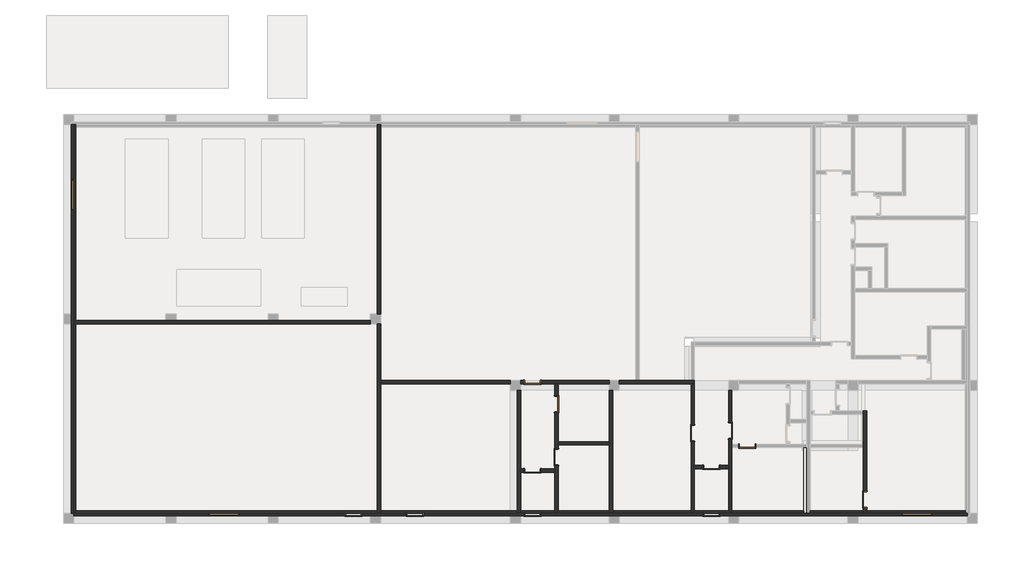
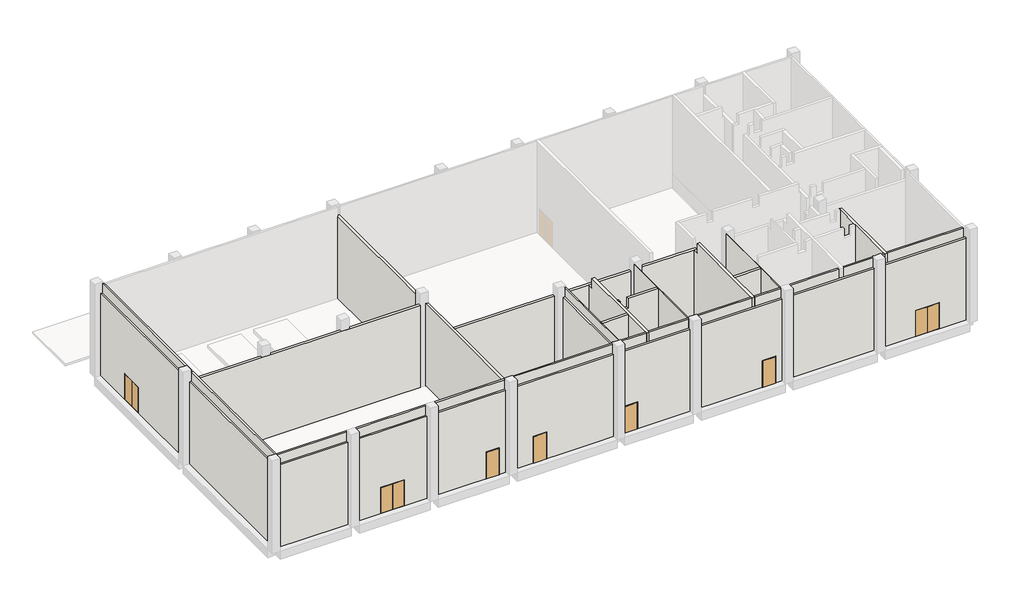
# One storey, part 1 of 4: 31 walls, 16 doors.
# Revit data of these elements (continued)
# Type "Double Door_Steel : H_DR_AR B12_Door_Double SD 02"
#   Type Mark = "FSD"
#   프레임 = ""
#   철물 = ""
#   유리/마감 = ""
#   위치/개소 = ""
#   부호 = "1/SD"
#   문번호 = ""
#   문기호 = "SD"
#   Analytic Construction = "<None>"
#   Height = 2100 mm
#   Width = 1800 mm
#   Define Thermal Properties by = 1
#   문 틀 = none
#   문 = none
#   Function = (empty or 0)
#   Assembly Code = ""
#   Wall Closure = (empty or 0)
# Type "Double Door_Steel : H_DR_AR B12_Door_Double FSD 02"
#   Type Mark = "FRD"
#   프레임 = ""
#   철물 = ""
#   유리/마감 = ""
#   위치/개소 = ""
#   부호 = "1/SD"
#   문번호 = ""
#   문기호 = "SD"
#   Analytic Construction = "<None>"
#   Height = 2100 mm
#   Width = 1800 mm
#   Define Thermal Properties by = 1
#   문 틀 = none
#   문 = none
#   Function = (empty or 0)
#   Assembly Code = ""
#   Wall Closure = (empty or 0)
# Type "Single Door_Steel : H_DR_AR B12_Door_Single FSD 01"
#   Type Mark = "FRD"
#   Analytic Construction = "<None>"
#   프레임 투영 외부. = 25 mm
#   프레임 투영 내부. = 25 mm
#   프레임 폭 = 75 mm
#   Height = 2160 mm
#   Width = 1020 mm
#   Define Thermal Properties by = 1
#   문 패널 = none
#   문 프레임 = none
#   Function = (empty or 0)
#   Wall Closure = (empty or 0)
# Type "H_WA_AR B02_Ext Wall RC-AG_EW5"
#   Type Comments = "AG"
#   Type Mark = "W1"
#   H_Rebar Ratio = 0.12
#   Layers, outside or top first: 0 mm no material (function 100); 0 mm no material (function 100); 150 mm no material (function 1); 0 mm no material (function 100); 0 mm no material (function 100); 0 mm no material (function 100)
# Type "H_WA_AR_B02_Ext Wall_RC_T200_W2"
#   Type Comments = "AG"
#   Type Mark = "W2"
#   H_Rebar Ratio = 0.12
#   Layers, outside or top first: 200 mm no material (function 1)
# Type "H_WA_AR B02_Int Wall MA_IW1 T200"
#   Type Comments = ""
#   Layers, outside or top first: 200 mm "00_Masonry_Conc. Block" (function 1)
# Type "H_WA_AR B02_Ext Wall DY-IN_EW1_VB"
#   Type Comments = "구조_콘크리트"
#   Layers, outside or top first: 126 mm "Rock Wool" (function 1)
# Element 1 (IfcDoor, "Double Door_Steel : H_DR_AR B12_Door_Double SD 02")
#   Frame Material = "ST"
#   H_Door Style Name = "Steel Door_Double_Normal_Fire Rating"
#   H_Door_Leaf = "ST"
#   H_Door_Vision = "-"
#   H_Door_Panic = "-"
#   H_Door_Style Remark = ""
#   H_Door_Type = "B1"
#   H_Door_Louver = "-"
#   H_Door Style No = 212_FSD_DD_N_F
#   Phase Created = New Construction
# Elements 2, 3 (IfcDoor, "Double Door_Steel : H_DR_AR B12_Door_Double FSD 02")
#   Frame Material = "ST"
#   H_Door Style Name = "Steel Door_Double_Normal_Fire Rating"
#   H_Door_Leaf = "ST"
#   H_Door_Vision = "-"
#   H_Door_Panic = "-"
#   H_Door_Style Remark = ""
#   H_Door_Type = "B1"
#   H_Door_Louver = "-"
#   H_Door Style No = 212_FSD_DD_N_F
#   Phase Created = New Construction
# Elements 4, 5, 6, 7, 8, 10, 11, 12, 13, 14, 15, 16 (IfcDoor, "Single Door_Steel : H_DR_AR B12_Door_Single FSD 01")
#   Frame Material = "ST"
#   H_Door Style Name = "Steel Door_Single_Normal_Fire Rating"
#   H_Door_Leaf = "ST"
#   H_Door_Vision = "-"
#   H_Door_Panic = "-"
#   H_Door_Style Remark = ""
#   H_Door_Type = "A1"
#   H_Door_Louver = "-"
#   H_Door Style No = 112_FSD_SD_N_F
#   Phase Created = New Construction
# Element 9 (IfcDoor, "Single Door_Steel : H_DR_AR B12_Door_Single FSD 01")
#   Frame Material = "WD"
#   H_Door Style Name = "Wood Door_Single_Normal"
#   H_Door_Leaf = "WD"
#   H_Door_Vision = "-"
#   H_Door_Panic = "-"
#   H_Door_Style Remark = ""
#   H_Door_Type = "A1"
#   H_Door_Louver = "-"
#   H_Door Style No = 181_WD_SD_N
#   Phase Created = New Construction
# Elements 17, 18 (IfcWall, "H_WA_AR B02_Ext Wall RC-AG_EW5")
#   H_Wall Style Name = "Concrete Wall+Acrylic Emulsion Paint on Fair Faced Concrete+Insulation"
#   H_Wall_Style Remark = ""
#   Top Offset = 0 mm
#   Base Offset = 0 mm
#   wall height = 7500.038 mm
#   H_Wall Style No = EW512A_CO
#   Phase Created = New Construction
#   Base Constraint = TOC(GF)
#   Top Constraint = TOC
#   Materials on its faces: "00_Concrete_Reinf. Conc."
# Elements 19, 20, 21 (IfcWall, "H_WA_AR_B02_Ext Wall_RC_T200_W2")
#   H_Wall Style Name = "Concrete Wall"
#   H_Wall_Style Remark = ""
#   Top Offset = 0 mm
#   Base Offset = 0 mm
#   wall height = 1000 mm
#   H_Wall Style No = IW311_CO
#   Phase Created = New Construction
#   Base Constraint = TOC(GF)
#   Top Constraint = TOC(GF-1)
#   Materials on its faces: "00_Concrete_Reinf. Conc."
# Elements 22, 23, 24, 25, 26, 27, 28, 29, 30, 31, 32, 33, 34, 35, 36 (IfcWall, "H_WA_AR B02_Int Wall MA_IW1 T200")
#   H_Wall Style Name = "Block Wall"
#   H_Wall_Style Remark = ""
#   Top Offset = 0 mm
#   Base Offset = 0 mm
#   wall height = 7500.038 mm
#   H_Wall Style No = IW211_BL
#   Phase Created = New Construction
#   Base Constraint = TOC(GF)
#   Top Constraint = TOC
#   Materials on its faces: "00_Masonry_Conc. Block"
# Elements 37, 38, 39, 40, 41, 42, 43, 44, 45, 46, 47 (IfcWall, "H_WA_AR B02_Ext Wall DY-IN_EW1_VB")
#   Top Offset = 0 mm
#   Base Offset = 0 mm
#   wall height = 7500.038 mm
#   Phase Created = New Construction
#   Base Constraint = TOC(GF)
#   Top Constraint = TOC
#   Materials on its faces: "Rock Wool"
# Materials
#   "00_Masonry_Conc. Block": class "Concrete", colour RGB 180 180 180, transparency 0, Description = "Conc. Block", Cost = 0, Image = Brick_Uniform_12inch_Running_Gray.png
#   "Rock Wool": class "Generic", colour RGB 120 120 120, transparency 0, Description = "Rock Wool", Cost = 0
#   "00_Concrete_Reinf. Conc.": class "Concrete", colour RGB 176 176 176, transparency 0, Description = "Reinf. Conc.", Cost = 0, Image = Concrete.Cast-In-Place.Flat.Polished.Grey.jpg
# Room at (9212.5, -2162.5) mm, phase "New Construction", upper level "TOC(GF)", upper offset 10500 mm, lower offset 0 mm
#   Comments = ""
#   Base Finish = "Epoxy Paint"
#   Ceiling Finish = "Acrylic Emulsion Paint"
#   Wall Finish = "Acrylic Emulsion Paint"
#   Floor Finish = "Epoxy Paint on Hardener Finish(Powder Type)"
#   Number = "101"
#   Name = "MECHANICAL ROOM"
#   H_Floor Base Material = "Concrete Slab"
#   H_Floor Finish Remark = "-"
#   H_Skirt Base Material = "Same as Wall"
#   H_Skirt Finish Remark = "-"
#   H_Wall Base Material = "Masonry Wall / Cement Plaster"
#   H_Wall Finish Remark = "-"
#   H_Ceiling Base Material = "Concrete Slab / Fair Faced Concrete"
#   H_Ceiling Finish Remark = "-"
#   Floor Finish Style No = FF331_HD_EP
#   Skirt Finish Style No = FB121_PA_EP
#   Wall Finish Style No = FW102_PA_AE
#   Ceiling Finish Style No = FC101_PA_AE
# Room at (9212.5, -13637.5) mm, phase "New Construction", upper level "TOC(GF)", upper offset 10500 mm, lower offset 0 mm
#   Comments = ""
#   Base Finish = "Epoxy Paint"
#   Ceiling Finish = "Acrylic Emulsion Paint"
#   Wall Finish = "Acrylic Emulsion Paint"
#   Floor Finish = "Non-Slip Epoxy Paint"
#   Number = "112"
#   Name = "ELECTRICAL ROOM(SS08)"
#   H_Floor Base Material = "Concrete Slab / Screed"
#   H_Floor Finish Remark = "-"
#   H_Skirt Base Material = "Same as Wall"
#   H_Skirt Finish Remark = "-"
#   H_Wall Base Material = "Masonry Wall / Cement Plaster"
#   H_Wall Finish Remark = "-"
#   H_Ceiling Base Material = "Concrete Slab / Fair Faced Concrete"
#   H_Ceiling Finish Remark = "-"
#   Floor Finish Style No = FF162_PA_EP
#   Skirt Finish Style No = FB121_PA_EP
#   Wall Finish Style No = FW102_PA_AE
#   Ceiling Finish Style No = FC101_PA_AE
# Room at (22300, -15387.5) mm, phase "New Construction", upper level "TOC(GF)", upper offset 10500 mm, lower offset 0 mm
#   Comments = ""
#   Base Finish = "Acid Resistant Ceramic Tile"
#   Ceiling Finish = "Acrylic Emulsion Paint"
#   Wall Finish = "Acid Resistant Paint"
#   Floor Finish = "Acid Resistant Ceramic Tile"
#   Number = "114"
#   Name = "BATTERY ROOM"
#   H_Floor Base Material = "Concrete Slab / Screed / Liquid Waterproofing"
#   H_Floor Finish Remark = "-"
#   H_Skirt Base Material = "Same as Wall"
#   H_Skirt Finish Remark = "-"
#   H_Wall Base Material = "Masonry Wall / Cement Plaster"
#   H_Wall Finish Remark = "-"
#   H_Ceiling Base Material = "Concrete Slab / Fair Faced Concrete"
#   H_Ceiling Finish Remark = "-"
#   Floor Finish Style No = FF222_TL_AC
#   Skirt Finish Style No = FB221_TL_AC
#   Wall Finish Style No = FW122_PA_AR
#   Ceiling Finish Style No = FC101_PA_AE
# Room at (49387.5, -3982.5) mm, phase "New Construction", upper level "TOC(GF)", upper offset 10500 mm, lower offset 0 mm
#   Comments = ""
#   Base Finish = "Coved Vinyl Tile"
#   Ceiling Finish = "Suspended Moisture Resistant Tiled Ceiling (M-Bar)"
#   Wall Finish = "Acrylic Emulsion Paint"
#   Floor Finish = "Vinyl Tile"
#   Number = "108"
#   Name = "BREAK ROOM"
#   H_Floor Base Material = "Concrete Slab / Screed"
#   H_Floor Finish Remark = "-"
#   H_Skirt Base Material = "Same as Wall"
#   H_Skirt Finish Remark = "-"
#   H_Wall Base Material = "Masonry Wall / Cement Plaster"
#   H_Wall Finish Remark = "-"
#   H_Ceiling Base Material = "Concrete Slab / Fair Faced Concrete"
#   H_Ceiling Finish Remark = "-"
#   H_Room H or CH = 2700 mm
#   Floor Finish Style No = FF232_TL_VN
#   Skirt Finish Style No = FB231_TL_VL
#   Wall Finish Style No = FW102_PA_AE
#   Ceiling Finish Style No = FC541_SC_MT
# Room at (50137.5, 912.5) mm, phase "New Construction", upper level "TOC(GF)", upper offset 10500 mm, lower offset 0 mm
#   Comments = ""
#   Base Finish = "Coved Vinyl Tile"
#   Ceiling Finish = "Suspended Acoustic Tiled Ceiling (M-Bar)"
#   Wall Finish = "Acrylic Emulsion Paint"
#   Floor Finish = "Vinyl Tile"
#   Number = "106"
#   Name = "SHIFT SUPERVISOR/DAY SUPERVISOR"
#   H_Floor Base Material = "Concrete Slab / Screed"
#   H_Floor Finish Remark = "-"
#   H_Skirt Base Material = "Same as Wall"
#   H_Skirt Finish Remark = "-"
#   H_Wall Base Material = "Masonry Wall / Cement Plaster"
#   H_Wall Finish Remark = "-"
#   H_Ceiling Base Material = "Concrete Slab / Fair Faced Concrete"
#   H_Ceiling Finish Remark = "-"
#   H_Room H or CH = 2700 mm
#   Floor Finish Style No = FF232_TL_VN
#   Skirt Finish Style No = FB231_TL_VL
#   Wall Finish Style No = FW102_PA_AE
#   Ceiling Finish Style No = FC531_SC_AT
# Room at (41100, -17262.5) mm, phase "New Construction", upper level "TOC(GF)", upper offset 10500 mm, lower offset 0 mm
#   Comments = ""
#   Base Finish = "Coved Ceramic Tile"
#   Ceiling Finish = "Suspended Moisture Resistant Tiled Ceiling (M-Bar)"
#   Wall Finish = "Glazed Ceramic Tile (≤2100) / Acrylic Emulsion Paint (>2100)"
#   Floor Finish = "Non-Slip Unglazed Ceramic Tile"
#   Number = "122"
#   Name = "TOILETS"
#   H_Floor Base Material = "Concrete Slab / Screed / Liquid Waterproofing"
#   H_Floor Finish Remark = "ex) 150x150x6T"
#   H_Skirt Base Material = "Same as Wall"
#   H_Skirt Finish Remark = "-"
#   H_Wall Base Material = "Masonry Wall"
#   H_Wall Finish Remark = ""
#   H_Ceiling Base Material = "Concrete Slab / Fair Faced Concrete"
#   H_Ceiling Finish Remark = "-"
#   H_Room H or CH = 2700 mm
#   Floor Finish Style No = FF202_TL_UC
#   Skirt Finish Style No = FB211_TL_CC
#   Wall Finish Style No = FW212C_TL_GC
#   Ceiling Finish Style No = FC541_SC_MT
# Room at (45050, -17262.5) mm, phase "New Construction", upper level "TOC(GF)", upper offset 10500 mm, lower offset 0 mm
#   Comments = ""
#   Base Finish = "Coved Vinyl Tile"
#   Ceiling Finish = "Suspended Acoustic Tiled Ceiling (M-Bar)"
#   Wall Finish = "Acrylic Emulsion Paint"
#   Floor Finish = "Vinyl Tile"
#   Number = "124"
#   Name = "STORE"
#   H_Floor Base Material = "Concrete Slab / Screed"
#   H_Floor Finish Remark = "-"
#   H_Skirt Base Material = "Same as Wall"
#   H_Skirt Finish Remark = "-"
#   H_Wall Base Material = "Masonry Wall / Cement Plaster"
#   H_Wall Finish Remark = "-"
#   H_Ceiling Base Material = "Concrete Slab / Fair Faced Concrete"
#   H_Ceiling Finish Remark = "-"
#   H_Room H or CH = 2700 mm
#   Floor Finish Style No = FF232_TL_VN
#   Skirt Finish Style No = FB231_TL_VL
#   Wall Finish Style No = FW102_PA_AE
#   Ceiling Finish Style No = FC531_SC_AT
# Room at (37700, -17887.5) mm, phase "New Construction", upper level "TOC(GF)", upper offset 10500 mm, lower offset 0 mm
#   Comments = ""
#   Base Finish = "Coved Vinyl Tile"
#   Ceiling Finish = "Suspended Acoustic Tiled Ceiling (M-Bar)"
#   Wall Finish = "Acrylic Emulsion Paint"
#   Floor Finish = "Vinyl Tile"
#   Number = "119"
#   Name = "AIR LOCK"
#   H_Floor Base Material = "Concrete Slab / Screed"
#   H_Floor Finish Remark = "-"
#   H_Skirt Base Material = "Same as Wall"
#   H_Skirt Finish Remark = "-"
#   H_Wall Base Material = "Masonry Wall / Cement Plaster"
#   H_Wall Finish Remark = "-"
#   H_Ceiling Base Material = "Concrete Slab / Fair Faced Concrete"
#   H_Ceiling Finish Remark = "-"
#   H_Room H or CH = 2700 mm
#   Floor Finish Style No = FF232_TL_VN
#   Skirt Finish Style No = FB231_TL_VL
#   Wall Finish Style No = FW102_PA_AE
#   Ceiling Finish Style No = FC531_SC_AT
# Room at (27500, -17987.5) mm, phase "New Construction", upper level "TOC(GF)", upper offset 10500 mm, lower offset 0 mm
#   Comments = ""
#   Base Finish = "Coved Vinyl Tile"
#   Ceiling Finish = "Suspended Acoustic Tiled Ceiling (M-Bar)"
#   Wall Finish = "Acrylic Emulsion Paint"
#   Floor Finish = "Vinyl Tile"
#   Number = "117"
#   Name = "AIR LOCK"
#   H_Floor Base Material = "Concrete Slab / Screed"
#   H_Floor Finish Remark = "-"
#   H_Skirt Base Material = "Same as Wall"
#   H_Skirt Finish Remark = "-"
#   H_Wall Base Material = "Masonry Wall / Cement Plaster"
#   H_Wall Finish Remark = "-"
#   H_Ceiling Base Material = "Concrete Slab / Fair Faced Concrete"
#   H_Ceiling Finish Remark = "-"
#   H_Room H or CH = 2700 mm
#   Floor Finish Style No = FF232_TL_VN
#   Skirt Finish Style No = FB231_TL_VL
#   Wall Finish Style No = FW102_PA_AE
#   Ceiling Finish Style No = FC531_SC_AT
# Room at (27500, -14100) mm, phase "New Construction", upper level "TOC(GF)", upper offset 10500 mm, lower offset 0 mm
#   Comments = ""
#   Base Finish = "Coved Vinyl Tile"
#   Ceiling Finish = "Suspended Acoustic Tiled Ceiling (M-Bar)"
#   Wall Finish = "Acrylic Emulsion Paint"
#   Floor Finish = "Vinyl Tile"
#   Number = "116"
#   Name = "CORRIDOR"
#   H_Floor Base Material = "Concrete Slab / Screed"
#   H_Floor Finish Remark = "-"
#   H_Skirt Base Material = "Same as Wall"
#   H_Skirt Finish Remark = "-"
#   H_Wall Base Material = "Masonry Wall / Cement Plaster"
#   H_Wall Finish Remark = "-"
#   H_Ceiling Base Material = "Concrete Slab / Fair Faced Concrete"
#   H_Ceiling Finish Remark = "-"
#   H_Room H or CH = 2700 mm
#   Floor Finish Style No = FF232_TL_VN
#   Skirt Finish Style No = FB231_TL_VL
#   Wall Finish Style No = FW102_PA_AE
#   Ceiling Finish Style No = FC531_SC_AT
# Room at (30200, -17187.5) mm, phase "New Construction", upper level "TOC(GF)", upper offset 10500 mm, lower offset 0 mm
#   Comments = ""
#   Base Finish = "Coved Vinyl Tile"
#   Ceiling Finish = "Acrylic Emulsion Paint"
#   Wall Finish = "2-COATS OF NON-CONDUCTIVE & FIRE RETARTDANT WITH COLOR PAINT"
#   Floor Finish = "Vinyl Tile"
#   Number = "115"
#   Name = "TELECOMS ROOM"
#   H_Floor Base Material = "Concrete Slab / Screed"
#   H_Floor Finish Remark = "-"
#   H_Skirt Base Material = "Same as Wall"
#   H_Skirt Finish Remark = "-"
#   H_Wall Base Material = "Masonry Wall / Cement Plaster"
#   H_Wall Finish Remark = ""
#   H_Ceiling Base Material = "Concrete Slab / Fair Faced Concrete"
#   H_Ceiling Finish Remark = "-"
#   Floor Finish Style No = FF232_TL_VN
#   Skirt Finish Style No = FB231_TL_VL
#   Wall Finish Style No = FW182_PA_CF
#   Ceiling Finish Style No = FC101_PA_AE
# Room at (49387.5, -8082.5) mm, phase "New Construction", upper level "TOC(GF)", upper offset 10500 mm, lower offset 0 mm
#   Comments = ""
#   Base Finish = "Coved Vinyl Tile"
#   Ceiling Finish = "Suspended Acoustic Tiled Ceiling (M-Bar)"
#   Wall Finish = "Acrylic Emulsion Paint"
#   Floor Finish = "Carpet Tile"
#   Number = "111"
#   Name = "PRAYER ROOM"
#   H_Floor Base Material = "Concrete Slab / Steel Trowel Finish"
#   H_Floor Finish Remark = "-"
#   H_Skirt Base Material = "Same as Wall"
#   H_Skirt Finish Remark = "-"
#   H_Wall Base Material = "Masonry Wall / Cement Plaster"
#   H_Wall Finish Remark = "-"
#   H_Ceiling Base Material = "Concrete Slab / Fair Faced Concrete"
#   H_Ceiling Finish Remark = "-"
#   H_Room H or CH = 2700 mm
#   Floor Finish Style No = FF275_TL_CA
#   Skirt Finish Style No = FB231_TL_VL
#   Wall Finish Style No = FW102_PA_AE
#   Ceiling Finish Style No = FC531_SC_AT
# Room at (30200, -13300) mm, phase "New Construction", upper level "TOC(GF)", upper offset 10500 mm, lower offset 0 mm
#   Comments = ""
#   Base Finish = "Coved Vinyl Tile"
#   Ceiling Finish = "Suspended Acoustic Tiled Ceiling (M-Bar)"
#   Wall Finish = "Acrylic Emulsion Paint"
#   Floor Finish = "Vinyl Tile"
#   Number = "113"
#   Name = "STORE"
#   H_Floor Base Material = "Concrete Slab / Screed"
#   H_Floor Finish Remark = "-"
#   H_Skirt Base Material = "Same as Wall"
#   H_Skirt Finish Remark = "-"
#   H_Wall Base Material = "Masonry Wall / Cement Plaster"
#   H_Wall Finish Remark = "-"
#   H_Ceiling Base Material = "Concrete Slab / Fair Faced Concrete"
#   H_Ceiling Finish Remark = "-"
#   H_Room H or CH = 2700 mm
#   Floor Finish Style No = FF232_TL_VN
#   Skirt Finish Style No = FB231_TL_VL
#   Wall Finish Style No = FW102_PA_AE
#   Ceiling Finish Style No = FC531_SC_AT
# Room at (34200, -15387.5) mm, phase "New Construction", upper level "TOC(GF)", upper offset 10500 mm, lower offset 0 mm
#   Comments = ""
#   Base Finish = "Coved Vinyl Tile"
#   Ceiling Finish = "Suspended Acoustic Tiled Ceiling (M-Bar)"
#   Wall Finish = "Acrylic Emulsion Paint"
#   Floor Finish = "Vinyl Tile"
#   Number = "118"
#   Name = "DRIVERS LOUNGE"
#   H_Floor Base Material = "Concrete Slab / Screed"
#   H_Floor Finish Remark = "-"
#   H_Skirt Base Material = "Same as Wall"
#   H_Skirt Finish Remark = "-"
#   H_Wall Base Material = "Masonry Wall / Cement Plaster"
#   H_Wall Finish Remark = "-"
#   H_Ceiling Base Material = "Concrete Slab / Fair Faced Concrete"
#   H_Ceiling Finish Remark = "-"
#   H_Room H or CH = 2700 mm
#   Floor Finish Style No = FF232_TL_VN
#   Skirt Finish Style No = FB231_TL_VL
#   Wall Finish Style No = FW102_PA_AE
#   Ceiling Finish Style No = FC531_SC_AT
# Room at (48937.5, -15387.5) mm, phase "New Construction", upper level "TOC(GF)", upper offset 10500 mm, lower offset 0 mm
#   Comments = ""
#   Base Finish = "Epoxy Paint"
#   Ceiling Finish = "Acrylic Emulsion Paint"
#   Wall Finish = "Acrylic Emulsion Paint"
#   Floor Finish = "Non-Slip Epoxy Paint with Epoxy Hardener"
#   Number = "125"
#   Name = "MAINTENANCE WORKSHOP"
#   H_Floor Base Material = "Concrete Slab / Steel Trowel Finish"
#   H_Floor Finish Remark = "-"
#   H_Skirt Base Material = "Same as Wall"
#   H_Skirt Finish Remark = "-"
#   H_Wall Base Material = "Masonry Wall / Cement Plaster"
#   H_Wall Finish Remark = "-"
#   H_Ceiling Base Material = "Concrete Slab / Fair Faced Concrete"
#   H_Ceiling Finish Remark = "-"
#   Floor Finish Style No = FF351_HD_EP
#   Skirt Finish Style No = FB121_PA_EP
#   Wall Finish Style No = FW102_PA_AE
#   Ceiling Finish Style No = FC101_PA_AE
# Room at (51435, -9900) mm, phase "New Construction", upper level "TOC(GF)", upper offset 10500 mm, lower offset 0 mm
#   Comments = ""
#   Base Finish = "Coved Ceramic Tile"
#   Ceiling Finish = "Suspended Moisture Resistant Tiled Ceiling (M-Bar)"
#   Wall Finish = "Glazed Ceramic Tile (≤2100) / Acrylic Emulsion Paint (>2100)"
#   Floor Finish = "Non-Slip Unglazed Ceramic Tile"
#   Number = "110"
#   Name = "ABLUTIONS"
#   H_Floor Base Material = "Concrete Slab / Screed / Liquid Waterproofing"
#   H_Floor Finish Remark = "ex) 150x150x6T"
#   H_Skirt Base Material = "Same as Wall"
#   H_Skirt Finish Remark = "-"
#   H_Wall Base Material = "Masonry Wall"
#   H_Wall Finish Remark = ""
#   H_Ceiling Base Material = "Concrete Slab / Fair Faced Concrete"
#   H_Ceiling Finish Remark = "-"
#   H_Room H or CH = 2700 mm
#   Floor Finish Style No = FF202_TL_UC
#   Skirt Finish Style No = FB211_TL_CC
#   Wall Finish Style No = FW212C_TL_GC
#   Ceiling Finish Style No = FC541_SC_MT
# Room at (43535, -10780.912) mm, phase "New Construction", upper level "TOC(GF)", upper offset 10500 mm, lower offset 0 mm
#   Comments = ""
#   Base Finish = "Coved Vinyl Tile"
#   Ceiling Finish = "Suspended Acoustic Tiled Ceiling (M-Bar)"
#   Wall Finish = "Acrylic Emulsion Paint"
#   Floor Finish = "Vinyl Tile"
#   Number = "120"
#   Name = "CORRIDOR"
#   H_Floor Base Material = "Concrete Slab / Screed"
#   H_Floor Finish Remark = "-"
#   H_Skirt Base Material = "Same as Wall"
#   H_Skirt Finish Remark = "-"
#   H_Wall Base Material = "Masonry Wall / Cement Plaster"
#   H_Wall Finish Remark = "-"
#   H_Ceiling Base Material = "Concrete Slab / Fair Faced Concrete"
#   H_Ceiling Finish Remark = "-"
#   H_Room H or CH = 2700 mm
#   Floor Finish Style No = FF232_TL_VN
#   Skirt Finish Style No = FB231_TL_VL
#   Wall Finish Style No = FW102_PA_AE
#   Ceiling Finish Style No = FC531_SC_AT
# Room at (44850, 2237.5) mm, phase "New Construction", upper level "TOC(GF)", upper offset 10500 mm, lower offset 0 mm
#   Comments = ""
#   Base Finish = "Coved Vinyl Tile"
#   Ceiling Finish = "Suspended Acoustic Tiled Ceiling (M-Bar)"
#   Wall Finish = "Acrylic Emulsion Paint"
#   Floor Finish = "Vinyl Tile"
#   Number = "104"
#   Name = "AIR LOCK"
#   H_Floor Base Material = "Concrete Slab / Screed"
#   H_Floor Finish Remark = "-"
#   H_Skirt Base Material = "Same as Wall"
#   H_Skirt Finish Remark = "-"
#   H_Wall Base Material = "Masonry Wall / Cement Plaster"
#   H_Wall Finish Remark = "-"
#   H_Ceiling Base Material = "Concrete Slab / Fair Faced Concrete"
#   H_Ceiling Finish Remark = "-"
#   H_Room H or CH = 2700 mm
#   Floor Finish Style No = FF232_TL_VN
#   Skirt Finish Style No = FB231_TL_VL
#   Wall Finish Style No = FW102_PA_AE
#   Ceiling Finish Style No = FC531_SC_AT
# Room at (47500, 1612.5) mm, phase "New Construction", upper level "TOC(GF)", upper offset 10500 mm, lower offset 0 mm
#   Comments = ""
#   Base Finish = "Coved Vinyl Tile"
#   Ceiling Finish = "Suspended Acoustic Tiled Ceiling (M-Bar)"
#   Wall Finish = "Acrylic Emulsion Paint"
#   Floor Finish = "Vinyl Tile"
#   Number = "105"
#   Name = "LIBRARY"
#   H_Floor Base Material = "Concrete Slab / Screed"
#   H_Floor Finish Remark = "-"
#   H_Skirt Base Material = "Same as Wall"
#   H_Skirt Finish Remark = "-"
#   H_Wall Base Material = "Masonry Wall / Cement Plaster"
#   H_Wall Finish Remark = "-"
#   H_Ceiling Base Material = "Concrete Slab / Fair Faced Concrete"
#   H_Ceiling Finish Remark = "-"
#   H_Room H or CH = 2700 mm
#   Floor Finish Style No = FF232_TL_VN
#   Skirt Finish Style No = FB231_TL_VL
#   Wall Finish Style No = FW102_PA_AE
#   Ceiling Finish Style No = FC531_SC_AT
# Room at (45600, -4225) mm, phase "New Construction", upper level "TOC(GF)", upper offset 10500 mm, lower offset 0 mm
#   Comments = ""
#   Base Finish = "Coved Vinyl Tile"
#   Ceiling Finish = "Suspended Acoustic Tiled Ceiling (M-Bar)"
#   Wall Finish = "Acrylic Emulsion Paint"
#   Floor Finish = "Vinyl Tile"
#   Number = "107"
#   Name = "CORRIDOR"
#   H_Floor Base Material = "Concrete Slab / Screed"
#   H_Floor Finish Remark = "-"
#   H_Skirt Base Material = "Same as Wall"
#   H_Skirt Finish Remark = "-"
#   H_Wall Base Material = "Masonry Wall / Cement Plaster"
#   H_Wall Finish Remark = "-"
#   H_Ceiling Base Material = "Concrete Slab / Fair Faced Concrete"
#   H_Ceiling Finish Remark = "-"
#   H_Room H or CH = 2700 mm
#   Floor Finish Style No = FF232_TL_VN
#   Skirt Finish Style No = FB231_TL_VL
#   Wall Finish Style No = FW102_PA_AE
#   Ceiling Finish Style No = FC531_SC_AT
# Room at (38525, -3912.5) mm, phase "New Construction", upper level "TOC(GF)", upper offset 10500 mm, lower offset 0 mm
#   Comments = ""
#   Base Finish = "Coved Vinyl Tile"
#   Ceiling Finish = "Suspended Acoustic Tiled Ceiling (M-Bar)"
#   Wall Finish = "Acrylic Emulsion Paint"
#   Floor Finish = "Anti-Dust Paint"
#   Number = "103"
#   Name = "CONTROL ROOM"
#   H_Floor Base Material = "Concrete Slab / Steel Trowel Finish"
#   H_Floor Finish Remark = "-"
#   H_Skirt Base Material = "Same as Wall"
#   H_Skirt Finish Remark = "-"
#   H_Wall Base Material = "Masonry Wall / Cement Plaster"
#   H_Wall Finish Remark = "-"
#   H_Ceiling Base Material = "Concrete Slab / Fair Faced Concrete"
#   H_Ceiling Finish Remark = "-"
#   H_Room H or CH = 3500 mm
#   Floor Finish Style No = FF151_PA_AD
#   Skirt Finish Style No = FB231_TL_VL
#   Wall Finish Style No = FW102_PA_AE
#   Ceiling Finish Style No = FC531_SC_AT
# Room at (25775, -3912.5) mm, phase "New Construction", upper level "TOC(GF)", upper offset 10500 mm, lower offset 0 mm
#   Comments = ""
#   Base Finish = "Coved Vinyl Tile"
#   Ceiling Finish = "Suspended Acoustic Tiled Ceiling (M-Bar)"
#   Wall Finish = "Acrylic Emulsion Paint"
#   Floor Finish = "Anti-Dust Paint"
#   Number = "102"
#   Name = "RACK ROOM"
#   H_Floor Base Material = "Concrete Slab / Steel Trowel Finish"
#   H_Floor Finish Remark = "-"
#   H_Skirt Base Material = "Same as Wall"
#   H_Skirt Finish Remark = "-"
#   H_Wall Base Material = "Masonry Wall / Cement Plaster"
#   H_Wall Finish Remark = "-"
#   H_Ceiling Base Material = "Concrete Slab / Fair Faced Concrete"
#   H_Ceiling Finish Remark = "-"
#   H_Room H or CH = 3000 mm
#   Floor Finish Style No = FF151_PA_AD
#   Skirt Finish Style No = FB231_TL_VL
#   Wall Finish Style No = FW102_PA_AE
#   Ceiling Finish Style No = FC531_SC_AT
# Room at (46975, -4790) mm, phase "New Construction", upper level "TOC(GF)", upper offset 10500 mm, lower offset 0 mm
#   Comments = ""
#   Base Finish = "Coved Ceramic Tile"
#   Ceiling Finish = "Suspended Moisture Resistant Tiled Ceiling (M-Bar)"
#   Wall Finish = "Glazed Ceramic Tile (≤2100) / Acrylic Emulsion Paint (>2100)"
#   Floor Finish = "Non-Slip Unglazed Ceramic Tile"
#   Number = "109"
#   Name = "JANITOR"
#   H_Floor Base Material = "Concrete Slab / Screed / Liquid Waterproofing"
#   H_Floor Finish Remark = "ex) 150x150x6T"
#   H_Skirt Base Material = "Same as Wall"
#   H_Skirt Finish Remark = "-"
#   H_Wall Base Material = "Masonry Wall"
#   H_Wall Finish Remark = ""
#   H_Ceiling Base Material = "Concrete Slab / Fair Faced Concrete"
#   H_Ceiling Finish Remark = "-"
#   H_Room H or CH = 2700 mm
#   Floor Finish Style No = FF202_TL_UC
#   Skirt Finish Style No = FB211_TL_CC
#   Wall Finish Style No = FW212C_TL_GC
#   Ceiling Finish Style No = FC541_SC_MT
# Room at (46500, -5480) mm, phase "New Construction", upper level "TOC(GF)", upper offset 10500 mm, lower offset 0 mm
#   Comments = ""
#   Base Finish = "Coved Vinyl Tile"
#   Ceiling Finish = "Suspended Acoustic Tiled Ceiling (M-Bar)"
#   Wall Finish = "Acrylic Emulsion Paint"
#   Floor Finish = "Vinyl Tile"
#   Number = "126"
#   Name = "EWH ROOM"
#   H_Floor Base Material = "Concrete Slab / Screed"
#   H_Floor Finish Remark = "-"
#   H_Skirt Base Material = "Same as Wall"
#   H_Skirt Finish Remark = "-"
#   H_Wall Base Material = "Masonry Wall / Cement Plaster"
#   H_Wall Finish Remark = "-"
#   H_Ceiling Base Material = "Concrete Slab / Fair Faced Concrete"
#   H_Ceiling Finish Remark = "-"
#   H_Room H or CH = 2700 mm
#   Floor Finish Style No = FF232_TL_VN
#   Skirt Finish Style No = FB231_TL_VL
#   Wall Finish Style No = FW102_PA_AE
#   Ceiling Finish Style No = FC531_SC_AT
# Room at (40500, -13375) mm, phase "New Construction", upper level "TOC(GF)", upper offset 10500 mm, lower offset 0 mm
#   Comments = ""
#   Base Finish = "Coved Ceramic Tile"
#   Ceiling Finish = "Suspended Moisture Resistant Tiled Ceiling (M-Bar)"
#   Wall Finish = "Glazed Ceramic Tile (≤2100) / Acrylic Emulsion Paint (>2100)"
#   Floor Finish = "Non-Slip Unglazed Ceramic Tile"
#   Number = "121"
#   Name = "LOCKER"
#   H_Floor Base Material = "Concrete Slab / Screed / Liquid Waterproofing"
#   H_Floor Finish Remark = "ex) 150x150x6T"
#   H_Skirt Base Material = "Same as Wall"
#   H_Skirt Finish Remark = "-"
#   H_Wall Base Material = "Masonry Wall"
#   H_Wall Finish Remark = ""
#   H_Ceiling Base Material = "Concrete Slab / Fair Faced Concrete"
#   H_Ceiling Finish Remark = "-"
#   H_Room H or CH = 2700 mm
#   Floor Finish Style No = FF202_TL_UC
#   Skirt Finish Style No = FB211_TL_CC
#   Wall Finish Style No = FW212C_TL_GC
#   Ceiling Finish Style No = FC541_SC_MT
# Room at (45050, -14275) mm, phase "New Construction", upper level "TOC(GF)", upper offset 10500 mm, lower offset 0 mm
#   Comments = ""
#   Base Finish = "Coved Vinyl Tile"
#   Ceiling Finish = "Suspended Acoustic Tiled Ceiling (M-Bar)"
#   Wall Finish = "Acrylic Emulsion Paint"
#   Floor Finish = "Vinyl Tile"
#   Number = "123"
#   Name = "STORE"
#   H_Floor Base Material = "Concrete Slab / Screed"
#   H_Floor Finish Remark = "-"
#   H_Skirt Base Material = "Same as Wall"
#   H_Skirt Finish Remark = "-"
#   H_Wall Base Material = "Masonry Wall / Cement Plaster"
#   H_Wall Finish Remark = "-"
#   H_Ceiling Base Material = "Concrete Slab / Fair Faced Concrete"
#   H_Ceiling Finish Remark = "-"
#   H_Room H or CH = 2700 mm
#   Floor Finish Style No = FF232_TL_VN
#   Skirt Finish Style No = FB231_TL_VL
#   Wall Finish Style No = FW102_PA_AE
#   Ceiling Finish Style No = FC531_SC_AT
# Room at (42800, -12649.619) mm, phase "New Construction", upper level "TOC(GF)", upper offset 10500 mm, lower offset 0 mm
#   Comments = ""
#   Base Finish = "Coved Ceramic Tile"
#   Ceiling Finish = "Suspended Moisture Resistant Tiled Ceiling (M-Bar)"
#   Wall Finish = "Glazed Ceramic Tile"
#   Floor Finish = "Non-Slip Unglazed Ceramic Tile"
#   Number = "127"
#   Name = "SHOWER ROOM"
#   H_Floor Base Material = "Concrete Slab / Screed / Liquid Waterproofing"
#   H_Floor Finish Remark = "ex) 150x150x6T"
#   H_Skirt Base Material = "Same as Wall"
#   H_Skirt Finish Remark = "-"
#   H_Wall Base Material = "Masonry Wall"
#   H_Wall Finish Remark = "-"
#   H_Ceiling Base Material = "Concrete Slab / Fair Faced Concrete"
#   H_Ceiling Finish Remark = "-"
#   H_Room H or CH = 2700 mm
#   Floor Finish Style No = FF202_TL_UC
#   Skirt Finish Style No = FB211_TL_CC
#   Wall Finish Style No = FW212_TL_GC
#   Ceiling Finish Style No = FC541_SC_MT
# Room at (42800, -14524.619) mm, phase "New Construction", upper level "TOC(GF)", upper offset 10500 mm, lower offset 0 mm
#   Comments = ""
#   Base Finish = "Coved Ceramic Tile"
#   Ceiling Finish = "Suspended Acoustic Tiled Ceiling (M-Bar)"
#   Wall Finish = "Acrylic Emulsion Paint"
#   Floor Finish = "Non-Slip Unglazed Ceramic Tile"
#   Number = "128"
#   Name = "EWH ROOM"
#   H_Floor Base Material = "Concrete Slab / Screed / Liquid Waterproofing"
#   H_Floor Finish Remark = "ex) 150x150x6T"
#   H_Skirt Base Material = "Same as Wall"
#   H_Skirt Finish Remark = "-"
#   H_Wall Base Material = "Masonry Wall / Cement Plaster"
#   H_Wall Finish Remark = "-"
#   H_Ceiling Base Material = "Concrete Slab / Fair Faced Concrete"
#   H_Ceiling Finish Remark = "-"
#   H_Room H or CH = 2700 mm
#   Floor Finish Style No = FF202_TL_UC
#   Skirt Finish Style No = FB211_TL_CC
#   Wall Finish Style No = FW102_PA_AE
#   Ceiling Finish Style No = FC531_SC_AT
